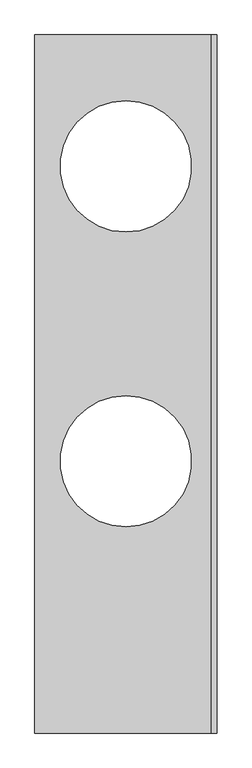
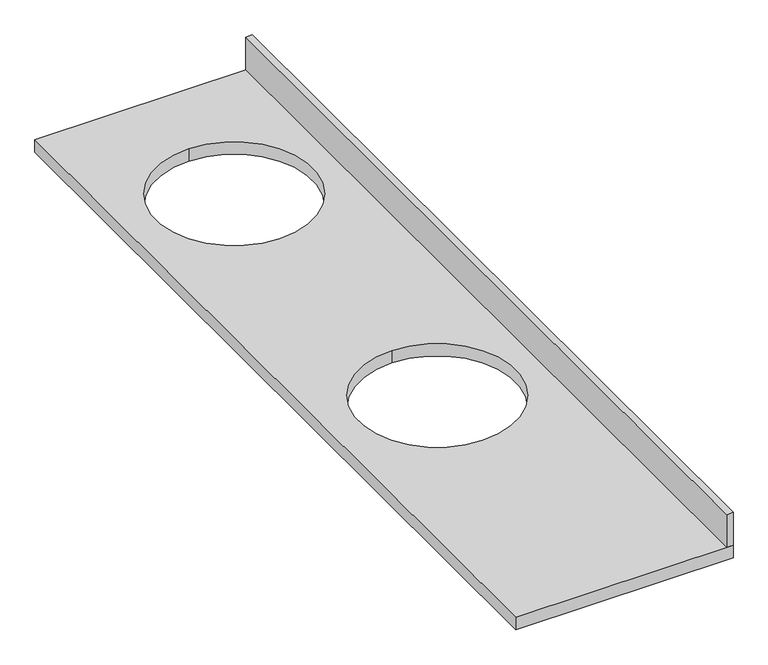
"""IFC4 building model written with IfcOpenShell, lengths in millimetres: furniture geometry."""

from ifc_helpers import new_model, si_unit, point, frame, frame_2d, origin, place, context, project, spatial, polyline, circle_curve, trimmed, segment, composite_curve, outline, extrude, source, transform, mapped, element, save


def furniture_ff69a8be(model_context):
    return source(origin(), model_context, "Body", "SweptSolid", [
        extrude(outline(polyline([(647741.6617239, -569560.2257591), (647760.7117239, -569560.2257591), (647760.7117239, -571990.2913841), (647741.6617239, -571990.2913841), (647741.6617239, -569560.2257591)])), frame((0.0, 0.0, 787.4), z_axis=(0.0, 0.0, 1.0), x_axis=(1.0, 0.0, 0.0)), (0.0, 0.0, 1.0), 101.6),
        extrude(outline(polyline([(647125.7117239, -571990.2913841), (647125.7117239, -569560.2257591), (647760.7117239, -569560.2257591), (647760.7117239, -571990.2913841), (647125.7117239, -571990.2913841)]), holes=[composite_curve([segment(trimmed(circle_curve(frame_2d((647443.2117239, -571044.1413841)), 228.6), [point((647443.2117239, -571272.7413841))], [point((647443.2117239, -570815.5413841))], True, "CARTESIAN"), True, "CONTINUOUS"), segment(trimmed(circle_curve(frame_2d((647443.2117239, -571044.1413841)), 228.6), [point((647443.2117239, -570815.5413841))], [point((647443.2117239, -571272.7413841))], True, "CARTESIAN"), True, "CONTINUOUS")], self_intersect=False), composite_curve([segment(trimmed(circle_curve(frame_2d((647443.2117239, -570017.4257591)), 228.6), [point((647443.2117239, -570246.0257591))], [point((647443.2117239, -569788.8257591))], True, "CARTESIAN"), True, "CONTINUOUS"), segment(trimmed(circle_curve(frame_2d((647443.2117239, -570017.4257591)), 228.6), [point((647443.2117239, -569788.8257591))], [point((647443.2117239, -570246.0257591))], True, "CARTESIAN"), True, "CONTINUOUS")], self_intersect=False)]), frame((0.0, 0.0, 749.3), z_axis=(0.0, 0.0, 1.0), x_axis=(1.0, 0.0, 0.0)), (0.0, 0.0, 1.0), 38.1),
    ])


if __name__ == "__main__":
    model = new_model("IFC4")
    model_context = context("Model", 3, world=origin())
    ifc_project = project(units=[si_unit("LENGTHUNIT", "METRE", prefix="MILLI")], contexts=[model_context])
    site = spatial("IfcSite", under=ifc_project)
    building = spatial("IfcBuilding", under=site)
    placement = place(None, origin())
    furniture_shape = furniture_ff69a8be(model_context)
    element("IfcFurniture", 1, ObjectType="Vanity Counter Top w 2 Round Sink Holes:72\":2442:72\":2442 : Vanity Counter Top w 2 Round Sink Holes:72\":2442:300472 : Vanity Counter Top w 2 Round Sink Holes:72\":2442:72\":2442 : Vanity Counter Top w 2 Round Sink Holes:72\":2442:300472", at=placement, inside=building, context=model_context, shape_type="MappedRepresentation", body=[
        mapped(furniture_shape, transform((0.0, 0.0, 0.0), x_axis=(1.0, 0.0, 0.0), y_axis=(0.0, 1.0, 0.0), z_axis=(0.0, 0.0, 1.0))),
    ])
    save(model, "model.ifc")

# Revit data of these elements
# Type "Vanity Counter Top w 2 Round Sink Holes:72\":2442:72\":2442 : Vanity Counter Top w 2 Round Sink Holes:72\":2442:300472 : Vanity Counter Top w 2 Round Sink Holes:72\":2442:72\":2442 : Vanity Counter Top w 2 Round Sink Holes:72\":2442:300472"
#   NameOverride = "Vanity Counter Top w 2 Round Sink Holes:72\":2442:72\":2442 : Vanity Counter Top w 2 Round Sink Holes:72\":2442:300472"
#   ObjectTypeOverride = "72\":2442 : Vanity Counter Top w 2 Round Sink Holes:72\":2442"
#   Tag = "300472"
# Element 1 (IfcFurniture, "Vanity Counter Top w 2 Round Sink Holes:72\":2442:72\":2442 : Vanity Counter Top w 2 Round Sink Holes:72\":2442:300472 : Vanity Counter Top w 2 Round Sink Holes:72\":2442:72\":2442 : Vanity Counter Top w 2 Round Sink Holes:72\":2442:300472")
#   Materials on its faces: "Counter Top"
# Materials
#   "Counter Top": class "Unassigned", colour RGB 226 177 128, transparency 0
